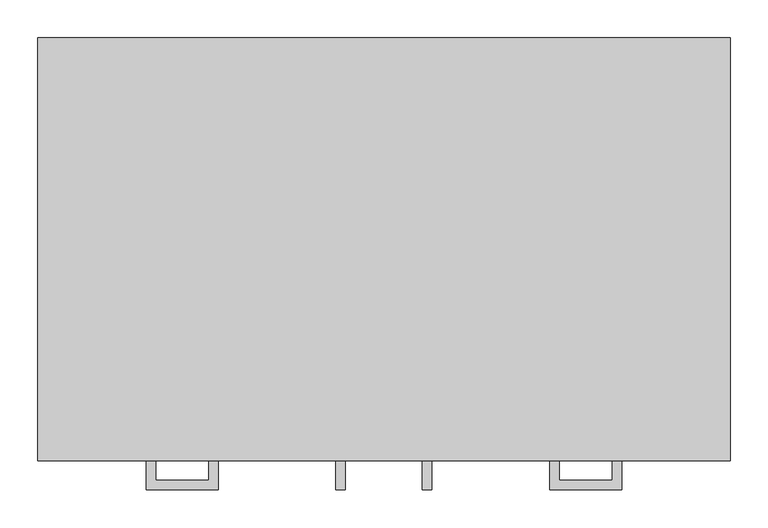
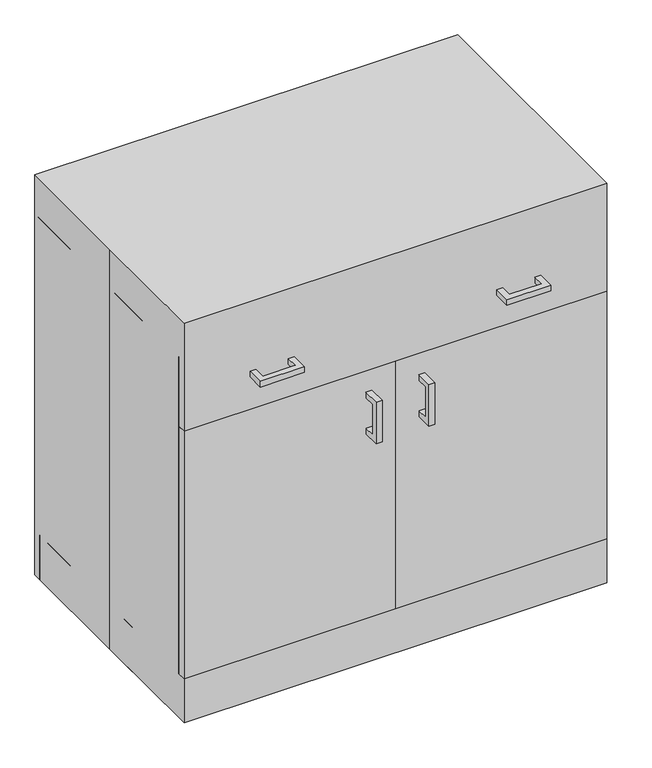
"""IFC4 building model written with IfcOpenShell, lengths in millimetres: proxy geometry, C04F0 - Cabinet, U-C-B, 1 Shelf, 2 Half DR, 2 DO, 36x36x22 : C04F0 - Cabinet, U-C-B, 1 Shelf, 2 Half DR, 2 DO, 36x36x22."""

from ifc_helpers import new_model, si_unit, frame, origin, origin_with_axes, place, context, project, spatial, polyline, outline, extrude, source, transform, mapped, element, save


def specialty_equipment_0dc6ae27(model_context):
    return source(origin(), model_context, "Body", "SweptSolid", [
        extrude(outline(polyline([(0.0, -279.4), (-457.2, -279.4), (-457.2, -260.35), (0.0, -260.35), (0.0, -279.4)])), frame((0.0, 0.0, 101.6), z_axis=(0.0, 0.0, 1.0), x_axis=(1.0, 0.0, 0.0)), (0.0, 0.0, 1.0), 565.15),
        extrude(outline(polyline([(-314.325, -317.5), (-314.325, -279.4), (-301.6409299, -279.4), (-301.6409299, -304.8159299), (-231.7590701, -304.8159299), (-231.7590701, -279.4), (-219.075, -279.4), (-219.075, -317.5), (-314.325, -317.5)])), frame((0.0, 0.0, 741.3462383), z_axis=(0.0, 0.0, 1.0), x_axis=(1.0, 0.0, 0.0)), (0.0, 0.0, 1.0), 12.7),
        extrude(outline(polyline([(314.325, -317.5), (219.075, -317.5), (219.075, -279.4), (231.7590701, -279.4), (231.7590701, -304.8159299), (301.6409299, -304.8159299), (301.6409299, -279.4), (314.325, -279.4), (314.325, -317.5)])), frame((0.0, 0.0, 741.3462383), z_axis=(0.0, 0.0, 1.0), x_axis=(1.0, 0.0, 0.0)), (0.0, 0.0, 1.0), 12.7),
        extrude(outline(polyline([(457.2, -279.4), (0.0, -279.4), (0.0, -260.35), (457.2, -260.35), (457.2, -279.4)])), frame((0.0, 0.0, 101.6), z_axis=(0.0, 0.0, 1.0), x_axis=(1.0, 0.0, 0.0)), (0.0, 0.0, 1.0), 565.15),
        extrude(outline(polyline([(-317.5, 523.8560937), (-317.5, 619.1060937), (-279.4, 619.1060937), (-279.4, 606.4220236), (-304.8159299, 606.4220236), (-304.8159299, 536.5401637), (-279.4, 536.5401637), (-279.4, 523.8560937), (-317.5, 523.8560937)])), frame((50.5065288, 0.0, 0.0), z_axis=(1.0, 0.0, 0.0), x_axis=(0.0, 1.0, 0.0)), (0.0, 0.0, 1.0), 12.7),
        extrude(outline(polyline([(-317.5, 523.8560937), (-317.5, 619.1060937), (-279.4, 619.1060937), (-279.4, 606.4220236), (-304.8159299, 606.4220236), (-304.8159299, 536.5401637), (-279.4, 536.5401637), (-279.4, 523.8560937), (-317.5, 523.8560937)])), frame((-63.7934712, 0.0, 0.0), z_axis=(1.0, 0.0, 0.0), x_axis=(0.0, 1.0, 0.0)), (0.0, 0.0, 1.0), 12.7),
        extrude(outline(polyline([(-457.2, 279.4), (457.2, 279.4), (457.2, -279.4), (-457.2, -279.4), (-457.2, 0.0), (-457.2, 279.4)])), origin_with_axes(), (0.0, 0.0, 1.0), 914.4),
        extrude(outline(polyline([(-457.2, -203.2), (-457.2, 260.35), (-438.15, 260.35), (-438.15, -203.2), (-457.2, -203.2)])), origin_with_axes(), (0.0, 0.0, 1.0), 101.6),
        extrude(outline(polyline([(438.15, -203.2), (438.15, 260.35), (457.2, 260.35), (457.2, -203.2), (438.15, -203.2)])), origin_with_axes(), (0.0, 0.0, 1.0), 101.6),
        extrude(outline(polyline([(438.15, -260.35), (438.15, 279.4), (457.2, 279.4), (457.2, -260.35), (438.15, -260.35)])), frame((0.0, 0.0, 101.6), z_axis=(0.0, 0.0, 1.0), x_axis=(1.0, 0.0, 0.0)), (0.0, 0.0, 1.0), 723.8674767),
        extrude(outline(polyline([(-457.2, -260.35), (-457.2, 279.4), (-438.15, 279.4), (-438.15, -260.35), (-457.2, -260.35)])), frame((0.0, 0.0, 101.6), z_axis=(0.0, 0.0, 1.0), x_axis=(1.0, 0.0, 0.0)), (0.0, 0.0, 1.0), 723.8674767),
        extrude(outline(polyline([(457.2, -279.4), (0.0, -279.4), (0.0, -260.35), (457.2, -260.35), (457.2, -279.4)])), frame((0.0, 0.0, 673.0674767), z_axis=(0.0, 0.0, 1.0), x_axis=(1.0, 0.0, 0.0)), (0.0, 0.0, 1.0), 152.4),
        extrude(outline(polyline([(0.0, -279.4), (-457.2, -279.4), (-457.2, -260.35), (0.0, -260.35), (0.0, -279.4)])), frame((0.0, 0.0, 673.0674767), z_axis=(0.0, 0.0, 1.0), x_axis=(1.0, 0.0, 0.0)), (0.0, 0.0, 1.0), 152.4),
        extrude(outline(polyline([(438.15, -203.2), (-438.15, -203.2), (-438.15, -184.15), (438.15, -184.15), (438.15, -203.2)])), origin_with_axes(), (0.0, 0.0, 1.0), 101.6),
        extrude(outline(polyline([(457.2, 260.35), (-457.2, 260.35), (-457.2, 279.4), (457.2, 279.4), (457.2, 260.35)])), origin_with_axes(), (0.0, 0.0, 1.0), 101.6),
        extrude(outline(polyline([(438.15, 260.35), (438.15, -260.35), (-438.15, -260.35), (-438.15, 260.35), (438.15, 260.35)])), frame((0.0, 0.0, 101.6), z_axis=(0.0, 0.0, 1.0), x_axis=(1.0, 0.0, 0.0)), (0.0, 0.0, 1.0), 19.1166954),
        extrude(outline(polyline([(438.15, 260.35), (-438.15, 260.35), (-438.15, 279.4), (438.15, 279.4), (438.15, 260.35)])), frame((0.0, 0.0, 101.6), z_axis=(0.0, 0.0, 1.0), x_axis=(1.0, 0.0, 0.0)), (0.0, 0.0, 1.0), 704.8174767),
    ])


if __name__ == "__main__":
    model = new_model("IFC4")
    model_context = context("Model", 3, world=origin())
    ifc_project = project(units=[si_unit("LENGTHUNIT", "METRE", prefix="MILLI")], contexts=[model_context])
    site = spatial("IfcSite", under=ifc_project)
    building = spatial("IfcBuilding", under=site)
    placement = place(None, origin())
    specialty_equipment_shape = specialty_equipment_0dc6ae27(model_context)
    element("IfcBuildingElementProxy", 1, Name="C04F0 - Cabinet, U-C-B, 1 Shelf, 2 Half DR, 2 DO, 36x36x22 : C04F0 - Cabinet, U-C-B, 1 Shelf, 2 Half DR, 2 DO, 36x36x22", ObjectType="C04F0 - Cabinet, U-C-B, 1 Shelf, 2 Half DR, 2 DO, 36x36x22 : C04F0 - Cabinet, U-C-B, 1 Shelf, 2 Half DR, 2 DO, 36x36x22", at=placement, inside=building, context=model_context, shape_type="MappedRepresentation", body=[
        mapped(specialty_equipment_shape, transform((0.0, 0.0, 0.0), x_axis=(1.0, 0.0, 0.0), y_axis=(0.0, 1.0, 0.0), z_axis=(0.0, 0.0, 1.0))),
    ])
    save(model, "model.ifc")

# Revit data of these elements
# Project information
#   Sheets - Total = "6"
#   Project Issue Date = "Issue Date"
#   Project Status = "Project Status"
#   Client Name = "Owner"
#   Project Address = "Enter address here"
#   Project Name = "Project Name"
#   Project Number = "Project Number"
#   Publication Date = "1-Feb-16"
# Type "C04F0 - Cabinet, U-C-B, 1 Shelf, 2 Half DR, 2 DO, 36x36x22 : C04F0 - Cabinet, U-C-B, 1 Shelf, 2 Half DR, 2 DO, 36x36x22"
#   Watts2 = "0"
#   Watts1 = "0"
#   Unit_Issue = "EA"
#   UTIL_6_Misc = "-"
#   UTIL_5_NonMedGas = "-"
#   UTIL_4_MiscGas = "-"
#   UTIL_3_MedGas = "-"
#   UTIL_2_Elec = "-"
#   UTIL_1_WaterDrain = "-"
#   Nomenclature = "Cabinet, U/C/B, 1 Shelf, 2 Half DR, 2 DO, 36x36x22"
#   NSN = "6530"
#   Location [instance default] = ""
#   JSN = "C04F0"
#   Fund_Source_VA = "-"
#   Fund_Source_Navy = "-"
#   Fund_Source_Army = "-"
#   Fund_Source_AF = "-"
#   ELEC_Volts2 = "0"
#   ELEC_Volts1 = "0"
#   ELEC_Phase2 = "0"
#   ELEC_Phase1 = "0"
#   ELEC_HertzSwitch = "0"
#   ELEC_HertzDependent = "0"
#   ELEC_Hertz = "0"
#   ELEC_Amps2 = "0"
#   ELEC_Amps1 = "0"
#   DetailDescription = "Standing height under counter base cabinet with an adjustable shelf and two half width drawers above solid hinged doors. Also referred to as a combination cabinet or a drawer and cupboard cabinet. For general purpose use throughout the facility."
#   CAT_VA = "A"
#   CAT_Navy = "A"
#   CAT_IHS = "-"
#   CAT_Army = "A"
#   CAT_AF = "A"
#   BTUperhour = "0"
#   Weight_IP = 135
#   DIM_Width_IP = 3' - 0"
#   DIM_Height_IP = 3' - 0"
#   DIM_Depth_IP = 1' - 10"
#   Top Panel Material = none
#   Toe Panel Material = none
#   Side Panel Material = none
#   Shelf Panel Material = none
#   Drawer Front Material = none
#   Door Panel Material = none
#   Back Panel Material = none
#   Assembly Code = ""
# Element 1 (IfcBuildingElementProxy, "C04F0 - Cabinet, U-C-B, 1 Shelf, 2 Half DR, 2 DO, 36x36x22 : C04F0 - Cabinet, U-C-B, 1 Shelf, 2 Half DR, 2 DO, 36x36x22")
#   Materials on its faces: "Default metal", "EquipSpace"
# Materials
#   "Default metal": class "Unassigned", colour RGB 204 204 204, transparency 0
#   "EquipSpace": class "Unassigned", colour RGB 221 217 195, transparency 0.5
